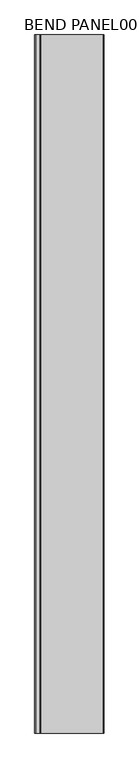
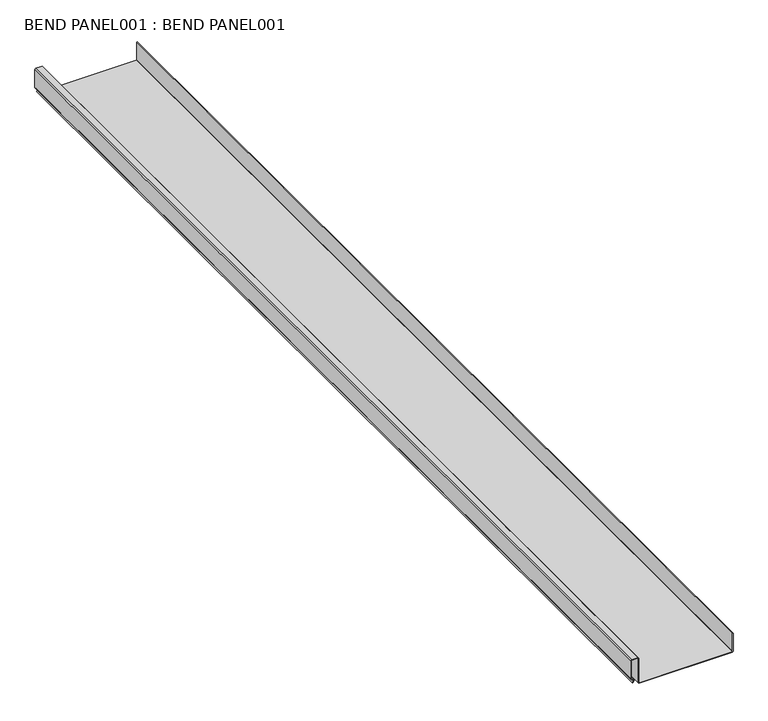
"""IFC4 building model written with IfcOpenShell, lengths in millimetres: proxy geometry, BEND PANEL001 : BEND PANEL001."""

from ifc_helpers import new_model, si_unit, frame, origin, place, context, project, spatial, polyline, outline, extrude, source, transform, mapped, element, save


def bend_panel001_bend_panel001_8c9d74ad(model_context):
    return source(origin(), model_context, "Body", "SweptSolid", [
        extrude(outline(polyline([(42589.7865091, 5848.1043867), (42589.2833292, 5849.1834595), (42594.3520112, 5851.5470247), (42596.210073, 5850.8707455), (42598.2005361, 5846.6022357), (42599.4643694, 5845.8020635), (42634.8859537, 5845.8020635), (42636.2841216, 5847.2002314), (42636.2841216, 5857.8984229), (42634.8859537, 5859.2965908), (42585.9088212, 5859.2965908), (42584.5106533, 5860.6947587), (42584.5106533, 6041.8377287), (42585.9101309, 6043.2372063), (42623.1706509, 6043.2372063), (42623.1706509, 6042.0465813), (42586.4033039, 6042.0465813), (42585.7012783, 6041.3445557), (42585.7012783, 5861.1879317), (42586.4019942, 5860.4872158), (42635.3791267, 5860.4872158), (42637.4747466, 5858.3915959), (42637.4747466, 5846.7070584), (42635.3791267, 5844.6114385), (42599.1191461, 5844.6114385), (42597.268896, 5845.7828894), (42595.3394273, 5849.920598), (42594.4082245, 5850.259528), (42589.7865091, 5848.1043867)])), frame((0.0, -1052.8906574, 0.0), z_axis=(0.0, 1.0, 0.0), x_axis=(0.0, 0.0, 1.0)), (0.0, 0.0, 1.0), 1999.85),
    ])


if __name__ == "__main__":
    model = new_model("IFC4")
    model_context = context("Model", 3, world=origin())
    ifc_project = project(units=[si_unit("LENGTHUNIT", "METRE", prefix="MILLI")], contexts=[model_context])
    site = spatial("IfcSite", under=ifc_project)
    building = spatial("IfcBuilding", under=site)
    placement = place(None, origin())
    bend_panel001_bend_panel001_shape = bend_panel001_bend_panel001_8c9d74ad(model_context)
    element("IfcBuildingElementProxy", 1, Name="BEND PANEL001 : BEND PANEL001", ObjectType="BEND PANEL001 : BEND PANEL001", at=placement, inside=building, context=model_context, shape_type="MappedRepresentation", body=[
        mapped(bend_panel001_bend_panel001_shape, transform((0.0, 0.0, 0.0), x_axis=(1.0, 0.0, 0.0), y_axis=(0.0, 1.0, 0.0), z_axis=(0.0, 0.0, 1.0))),
    ])
    save(model, "model.ifc")

# Revit data of these elements
# Type "BEND PANEL001 : BEND PANEL001"
#   NameOverride = "BEND PANEL001"
# Element 1 (IfcBuildingElementProxy, "BEND PANEL001 : BEND PANEL001")
#   Materials on its faces: "STANDING SEAM METAL ROOF FOLLOW MANU. RECOMMENDED EDGE/TRANSITION DETAILS"
# Materials
#   "STANDING SEAM METAL ROOF FOLLOW MANU. RECOMMENDED EDGE/TRANSITION DETAILS": class "Unassigned", colour RGB 128 128 128, transparency 0, Cost = 0
